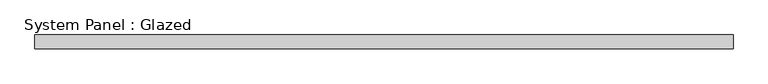
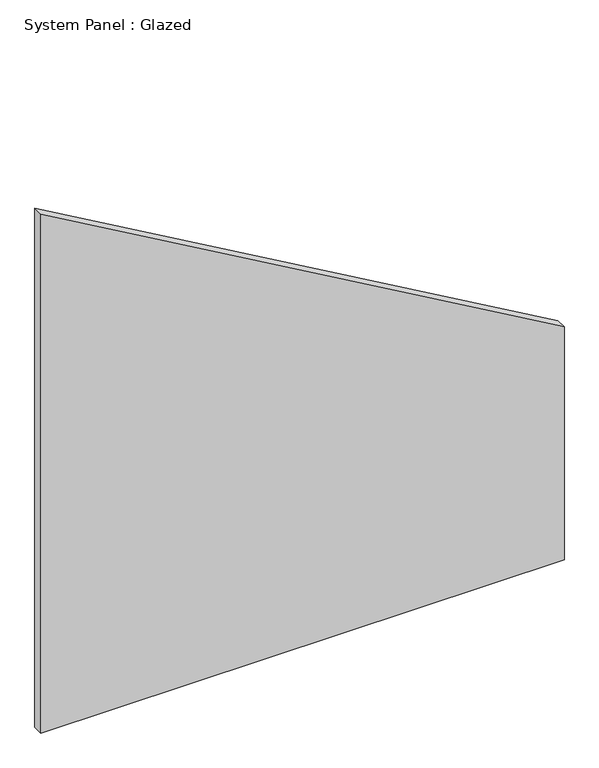
"""IFC4 building model written with IfcOpenShell, lengths in millimetres: plate geometry, System Panel : Glazed."""

import ifcopenshell
import ifcopenshell.guid

model = None  # the IFC model being written
_history = None  # IfcOwnerHistory: only IFC2X3 demands one
_inside = {}  # id of a spatial element -> (the spatial element, [elements in it])
_under = {}  # id of a project, library or spatial element -> (it, [spatial elements below it])
_declared = {}  # id of a project -> (the project, [libraries it declares])
_typed = {}  # id of a type object -> (the type object, [elements of that type])
_made_of = {}  # id of a material, layer set ... -> (it, [elements and type objects made of it])


def new_model(schema):
    """Start an empty IFC model of exactly this schema.

    Asked for "IFC4X3", IfcOpenShell would pick the latest addendum, in which some entities
    have other attributes; the version numbers below select the first issue.
    IFC2X3 requires an IfcOwnerHistory on every rooted entity: one is made here for all.
    """
    global model, _history
    if schema == "IFC4X3":
        model = ifcopenshell.file(schema_version=(4, 3, 0, 0))
    else:
        model = ifcopenshell.file(schema=schema)
    _inside.clear()
    _under.clear()
    _declared.clear()
    _typed.clear()
    _made_of.clear()
    _history = None
    if model.schema == "IFC2X3":
        org = make("IfcOrganization", Name="unknown")
        user = make(
            "IfcPersonAndOrganization",
            ThePerson=make("IfcPerson", FamilyName="unknown"),
            TheOrganization=org,
        )
        app = make(
            "IfcApplication",
            ApplicationDeveloper=org,
            Version="unknown",
            ApplicationFullName="unknown",
            ApplicationIdentifier="unknown",
        )
        _history = make(
            "IfcOwnerHistory",
            OwningUser=user,
            OwningApplication=app,
            ChangeAction="ADDED",
            CreationDate=0,
        )
    return model


def make(cls, **values):
    """One entity of the class cls with the attributes given. An attribute that is None is left unset."""
    return model.create_entity(
        cls, **{name: value for name, value in values.items() if value is not None}
    )


def rooted(cls, **values):
    """An entity with a GlobalId (a new one), such as an element, a storey or a relation."""
    return make(cls, GlobalId=ifcopenshell.guid.new(), OwnerHistory=_history, **values)


def si_unit(unit_type, name, prefix=None):
    """IfcSIUnit, for example si_unit("LENGTHUNIT", "METRE", prefix="MILLI")."""
    return make("IfcSIUnit", UnitType=unit_type, Prefix=prefix, Name=name)


def assignment(units):
    """IfcUnitAssignment: the units of a project."""
    return None if units is None else make("IfcUnitAssignment", Units=units)


def point(xyz):
    """IfcCartesianPoint."""
    return None if xyz is None else make("IfcCartesianPoint", Coordinates=xyz)


def direction(xyz):
    """IfcDirection."""
    return None if xyz is None else make("IfcDirection", DirectionRatios=xyz)


def frame(location, z_axis=None, x_axis=None):
    """IfcAxis2Placement3D, a coordinate frame: its origin and axes. An axis left out is left unset."""
    return make(
        "IfcAxis2Placement3D",
        Location=point(location),
        Axis=direction(z_axis),
        RefDirection=direction(x_axis),
    )


def origin():
    """The frame at (0, 0, 0) with its axes left unset."""
    return frame((0.0, 0.0, 0.0))


def place(relative_to, where):
    """IfcLocalPlacement: puts the frame where relative to a parent placement (None: the world)."""
    return make(
        "IfcLocalPlacement", PlacementRelTo=relative_to, RelativePlacement=where
    )


def context(
    kind, dimensions, precision=None, world=None, true_north=None, identifier=None
):
    """IfcGeometricRepresentationContext, for example the 3D "Model" context."""
    return make(
        "IfcGeometricRepresentationContext",
        ContextIdentifier=identifier,
        ContextType=kind,
        CoordinateSpaceDimension=dimensions,
        Precision=precision,
        WorldCoordinateSystem=world,
        TrueNorth=true_north,
    )


def project(units=None, contexts=None):
    """IfcProject with its units and contexts."""
    return rooted(
        "IfcProject",
        Name="project",
        RepresentationContexts=contexts,
        UnitsInContext=assignment(units),
    )


def spatial(cls, under=None, at=None, **own):
    """A site, building, storey or space (cls), placed at a placement, below another one or the project."""
    s = rooted(cls, ObjectPlacement=at, **own)
    if under is not None:
        _under.setdefault(under.id(), (under, []))[1].append(s)
    return s


def polyline(points):
    """IfcPolyline through the points."""
    return make("IfcPolyline", Points=[point(p) for p in points])


def outline(outer, holes=None, kind="AREA"):
    """IfcArbitraryClosedProfileDef: a profile drawn as a closed curve; with holes, ...WithVoids."""
    if holes is None:
        return make("IfcArbitraryClosedProfileDef", ProfileType=kind, OuterCurve=outer)
    return make(
        "IfcArbitraryProfileDefWithVoids",
        ProfileType=kind,
        OuterCurve=outer,
        InnerCurves=holes,
    )


def extrude(swept, where, along, depth):
    """IfcExtrudedAreaSolid: the profile swept, set in the frame where, extruded along a direction by depth."""
    return make(
        "IfcExtrudedAreaSolid",
        SweptArea=swept,
        Position=where,
        ExtrudedDirection=direction(along),
        Depth=depth,
    )


def shape(context_of_items, identifier, shape_type, items):
    """IfcShapeRepresentation: the items that make up one representation, for example the "Body"."""
    return make(
        "IfcShapeRepresentation",
        ContextOfItems=context_of_items,
        RepresentationIdentifier=identifier,
        RepresentationType=shape_type,
        Items=items,
    )


def source(mapping_origin, context_of_items, identifier, shape_type, items):
    """IfcRepresentationMap: a shape defined once, which mapped items show again and again."""
    return make(
        "IfcRepresentationMap",
        MappingOrigin=mapping_origin,
        MappedRepresentation=shape(context_of_items, identifier, shape_type, items),
    )


def transform(
    local_origin,
    x_axis=None,
    y_axis=None,
    z_axis=None,
    scale=None,
    scale2=None,
    scale3=None,
    uniform=True,
):
    """IfcCartesianTransformationOperator3D, or its non-uniform kind. x_axis, y_axis, z_axis: its Axis1, 2, 3."""
    if uniform:
        return make(
            "IfcCartesianTransformationOperator3D",
            Axis1=direction(x_axis),
            Axis2=direction(y_axis),
            LocalOrigin=point(local_origin),
            Scale=scale,
            Axis3=direction(z_axis),
        )
    return make(
        "IfcCartesianTransformationOperator3DnonUniform",
        Axis1=direction(x_axis),
        Axis2=direction(y_axis),
        LocalOrigin=point(local_origin),
        Scale=scale,
        Axis3=direction(z_axis),
        Scale2=scale2,
        Scale3=scale3,
    )


def mapped(mapping_source, mapping_target):
    """IfcMappedItem: shows the shape of a source again, moved by a transform."""
    return make(
        "IfcMappedItem", MappingSource=mapping_source, MappingTarget=mapping_target
    )


def made_of(thing, what):
    """Note that an element or type object is made of a material, layer set ...; save() writes the relation."""
    if what is not None:
        _made_of.setdefault(what.id(), (what, []))[1].append(thing)
    return thing


def element(
    cls,
    number,
    at=None,
    inside=None,
    cuts=None,
    type_object=None,
    material=None,
    context=None,
    identifier="Body",
    shape_type=None,
    held_by="IfcProductDefinitionShape",
    body=None,
    shapes=None,
    **own,
):
    """One element of the class cls, such as IfcWall. Its Tag is "e" and its number.

    at: its placement. inside: the storey or other place that contains it. cuts: it is an
    opening in that element (IfcRelVoidsElement). A single representation is given by context,
    identifier, shape_type and body (its items); several are given by shapes. held_by: the class
    of the entity that holds the representations. save() writes the other relations.
    """
    e = rooted(cls, Tag="e%d" % number, ObjectPlacement=at, **own)
    if body is not None:
        shapes = [shape(context, identifier, shape_type, body)]
    if shapes is not None:
        e.Representation = make(held_by, Representations=shapes)
    if inside is not None:
        _inside.setdefault(inside.id(), (inside, []))[1].append(e)
    if cuts is not None:
        rooted(
            "IfcRelVoidsElement", RelatingBuildingElement=cuts, RelatedOpeningElement=e
        )
    if type_object is not None:
        _typed.setdefault(type_object.id(), (type_object, []))[1].append(e)
    return made_of(e, material)


def aggregate(whole, parts):
    """IfcRelAggregates: a whole, such as a stair, and the parts it consists of."""
    return rooted("IfcRelAggregates", RelatingObject=whole, RelatedObjects=parts)


def save(model, path):
    """Write the relations noted so far, then the file.

    IfcRelAggregates (storeys below a building ...), IfcRelContainedInSpatialStructure (elements
    in a storey), IfcRelDefinesByType, IfcRelAssociatesMaterial and IfcRelDeclares: one each for
    every whole, place, type object, material and project.
    """
    for whole, parts in _under.values():
        aggregate(whole, parts)
    for where, things in _inside.values():
        rooted(
            "IfcRelContainedInSpatialStructure",
            RelatedElements=things,
            RelatingStructure=where,
        )
    for kind, things in _typed.values():
        rooted("IfcRelDefinesByType", RelatedObjects=things, RelatingType=kind)
    for what, things in _made_of.values():
        rooted("IfcRelAssociatesMaterial", RelatedObjects=things, RelatingMaterial=what)
    for by, libraries in _declared.values():
        rooted("IfcRelDeclares", RelatingContext=by, RelatedDefinitions=libraries)
    model.write(path)


def system_panel_glazed_62c7097b(model_context):
    return source(origin(), model_context, "Body", "SweptSolid", [
        extrude(outline(polyline([(0.0, -626.7857144), (0.0, 626.7857144), (589.5081595, 626.7857144), (1313.2579614, -626.7857144), (0.0, -626.7857144)])), frame((0.0, 24.5, 0.0), z_axis=(0.0, 1.0, 0.0), x_axis=(0.0, 0.0, 1.0)), (0.0, 0.0, 1.0), 25.0),
    ])


if __name__ == "__main__":
    model = new_model("IFC4")
    model_context = context("Model", 3, world=origin())
    ifc_project = project(units=[si_unit("LENGTHUNIT", "METRE", prefix="MILLI")], contexts=[model_context])
    site = spatial("IfcSite", under=ifc_project)
    building = spatial("IfcBuilding", under=site)
    placement = place(None, origin())
    system_panel_glazed_shape = system_panel_glazed_62c7097b(model_context)
    element("IfcPlate", 1, ObjectType="System Panel : Glazed", at=placement, inside=building, context=model_context, shape_type="MappedRepresentation", body=[
        mapped(system_panel_glazed_shape, transform((0.0, 0.0, 0.0), x_axis=(1.0, 0.0, 0.0), y_axis=(0.0, 1.0, 0.0), z_axis=(0.0, 0.0, 1.0))),
    ])
    save(model, "model.ifc")

# Revit data of these elements
# Type "System Panel : Glazed"
#   Construction Type Id = "GSP4R"
#   Analytic Construction = "1/8 in Pilkington single glazing"
#   Visual Light Transmittance = 0.9
#   Solar Heat Gain Coefficient = 0.86
#   Heat Transfer Coefficient (U) = 6.7069 W/(m²·K)
#   Define Thermal Properties by = 1
# Element 1 (IfcPlate, "System Panel : Glazed")
#   Materials on its faces: "Glass"
# Materials
#   "Glass": class "Glass", colour RGB 0 128 192, transparency 0.75, Description = "Soda Lime Glass", Cost = 0
